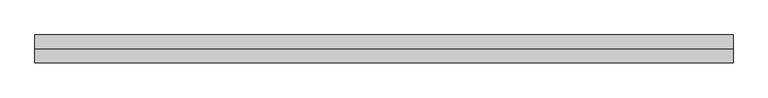
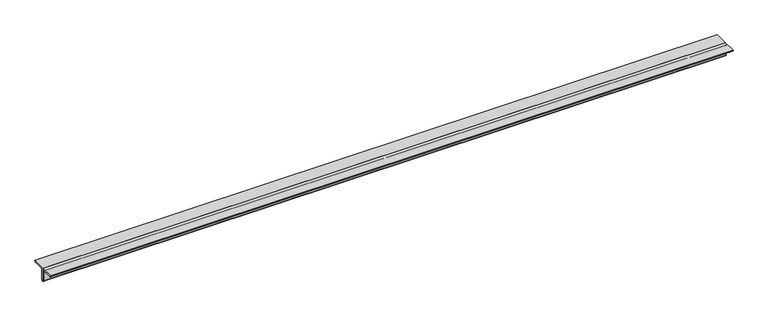
"""IFC4 building model written with IfcOpenShell, lengths in millimetres: member geometry, Steel Framing_2Ls_KS : H_SB_AR_S02_2Ls-100x100x10_VBR1."""

from ifc_helpers import new_model, si_unit, point, frame, frame_2d, origin, place, context, project, spatial, polyline, circle_curve, trimmed, segment, composite_curve, outline, extrude, source, transform, mapped, element, save


def member_6a50da69(model_context):
    return source(origin(), model_context, "Body", "SweptSolid", [
        extrude(outline(composite_curve([segment(polyline([(0.0, 28.2), (100.0, 28.2)]), True, "CONTINUOUS"), segment(trimmed(circle_curve(frame_2d((90.0, 28.2)), 10.0), [point((100.0, 28.2))], [point((90.0, 18.2))], False, "CARTESIAN"), True, "CONTINUOUS"), segment(polyline([(90.0, 18.2), (20.0, 18.2)]), True, "CONTINUOUS"), segment(trimmed(circle_curve(frame_2d((20.0, 8.2)), 10.0), [point((20.0, 18.2))], [point((10.0, 8.2))], True, "CARTESIAN"), True, "CONTINUOUS"), segment(polyline([(10.0, 8.2), (10.0, -61.8)]), True, "CONTINUOUS"), segment(trimmed(circle_curve(frame_2d((0.0, -61.8)), 10.0), [point((10.0, -61.8))], [point((0.0, -71.8))], False, "CARTESIAN"), True, "CONTINUOUS"), segment(polyline([(0.0, -71.8), (0.0, 28.2)]), True, "CONTINUOUS")], self_intersect=False)), frame((-2590.3354834, 0.0, 0.0), z_axis=(1.0, 0.0, 0.0), x_axis=(0.0, 1.0, 0.0)), (0.0, 0.0, 1.0), 5034.8971694),
        extrude(outline(composite_curve([segment(polyline([(0.0, 28.2), (0.0, -71.8)]), True, "CONTINUOUS"), segment(trimmed(circle_curve(frame_2d((0.0, -61.8)), 10.0), [point((0.0, -71.8))], [point((-10.0, -61.8))], False, "CARTESIAN"), True, "CONTINUOUS"), segment(polyline([(-10.0, -61.8), (-10.0, 8.2)]), True, "CONTINUOUS"), segment(trimmed(circle_curve(frame_2d((-20.0, 8.2)), 10.0), [point((-10.0, 8.2))], [point((-20.0, 18.2))], True, "CARTESIAN"), True, "CONTINUOUS"), segment(polyline([(-20.0, 18.2), (-90.0, 18.2)]), True, "CONTINUOUS"), segment(trimmed(circle_curve(frame_2d((-90.0, 28.2)), 10.0), [point((-90.0, 18.2))], [point((-100.0, 28.2))], False, "CARTESIAN"), True, "CONTINUOUS"), segment(polyline([(-100.0, 28.2), (0.0, 28.2)]), True, "CONTINUOUS")], self_intersect=False)), frame((-2590.3354834, 0.0, 0.0), z_axis=(1.0, 0.0, 0.0), x_axis=(0.0, 1.0, 0.0)), (0.0, 0.0, 1.0), 5034.8971694),
    ])


if __name__ == "__main__":
    model = new_model("IFC4")
    model_context = context("Model", 3, world=origin())
    ifc_project = project(units=[si_unit("LENGTHUNIT", "METRE", prefix="MILLI")], contexts=[model_context])
    site = spatial("IfcSite", under=ifc_project)
    building = spatial("IfcBuilding", under=site)
    placement = place(None, origin())
    member_shape = member_6a50da69(model_context)
    element("IfcMember", 1, ObjectType="Steel Framing_2Ls_KS : H_SB_AR_S02_2Ls-100x100x10_VBR1", at=placement, inside=building, context=model_context, shape_type="MappedRepresentation", body=[
        mapped(member_shape, transform((0.0, 0.0, 0.0), x_axis=(1.0, 0.0, 0.0), y_axis=(0.0, 1.0, 0.0), z_axis=(0.0, 0.0, 1.0))),
    ])
    save(model, "model.ifc")

# Revit data of these elements
# Type "Steel Framing_2Ls_KS : H_SB_AR_S02_2Ls-100x100x10_VBR1"
#   Type Comments = "MAIN"
#   Type Mark = "VBR1"
#   H_SectionID = "2Ls-100x100x10"
#   Assembly Code = "B10"
#   Legs = "LLBB"
#   H_Ratio for Additional Steel Plate = 0.2
#   W = 0
#   Perimeter = 0.80 m²/m
#   Nominal Weight = 29.80 kgf/m
#   Length [instance default] = 1524 mm
#   Space = 0 mm
#   b = 100 mm
#   d = 100 mm
#   t = 10 mm
#   y = 28.2 mm
#   A = 0.0038 m²
#   Structural Material [instance default] = Steel, 45-345
# Element 1 (IfcMember, "Steel Framing_2Ls_KS : H_SB_AR_S02_2Ls-100x100x10_VBR1")
#   Materials on its faces: "Steel, 45-345"
# Materials
#   "Steel, 45-345": class "Metal", colour RGB 189 187 185, transparency 0, Description = "Steel 345 MPa", Cost = 0
